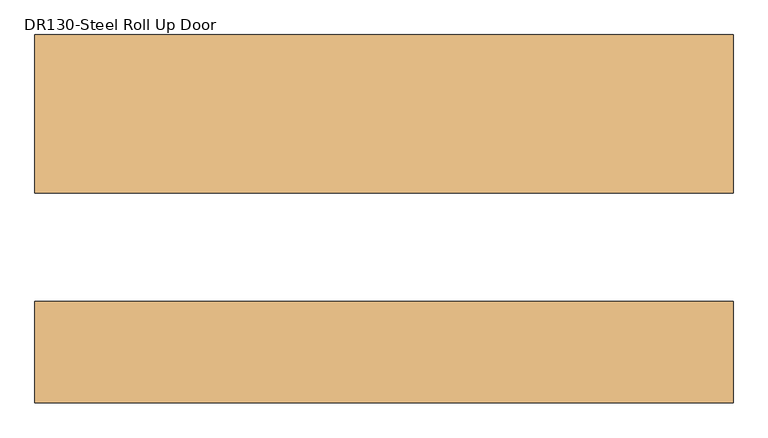
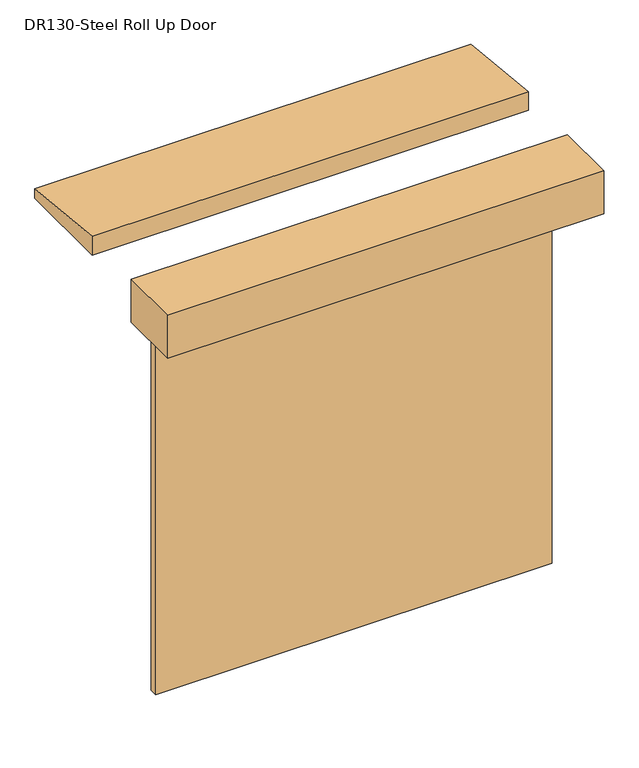
"""IFC4 building model written with IfcOpenShell, lengths in millimetres: door geometry, DR130-Steel Roll Up Door : DR131-Steel Roll Up Door-W4000xH4000mm."""

from ifc_helpers import new_model, si_unit, frame, origin, origin_with_axes, place, context, project, spatial, polyline, outline, extrude, source, transform, mapped, element, save


def dr130_steel_roll_up_door_abb043e2(model_context):
    return source(origin(), model_context, "Body", "SweptSolid", [
        extrude(outline(polyline([(1175.0, 4300.0), (175.0, 4300.0), (175.0, 4500.0), (1175.0, 4400.0), (1175.0, 4300.0)])), frame((-2203.2, 0.0, 0.0), z_axis=(1.0, 0.0, 0.0), x_axis=(0.0, 1.0, 0.0)), (0.0, 0.0, 1.0), 4406.4),
        extrude(outline(polyline([(2203.2, -1148.8), (-2203.2, -1148.8), (-2203.2, -510.0), (2203.2, -510.0), (2203.2, -1148.8)])), frame((0.0, 0.0, 4000.0), z_axis=(0.0, 0.0, 1.0), x_axis=(1.0, 0.0, 0.0)), (0.0, 0.0, 1.0), 457.2),
        extrude(outline(polyline([(2000.0, -510.0), (2000.0, -590.0), (-2000.0, -590.0), (-2000.0, -510.0), (2000.0, -510.0)])), origin_with_axes(), (0.0, 0.0, 1.0), 4000.0),
    ])


if __name__ == "__main__":
    model = new_model("IFC4")
    model_context = context("Model", 3, world=origin())
    ifc_project = project(units=[si_unit("LENGTHUNIT", "METRE", prefix="MILLI")], contexts=[model_context])
    site = spatial("IfcSite", under=ifc_project)
    building = spatial("IfcBuilding", under=site)
    placement = place(None, origin())
    dr130_steel_roll_up_door_shape = dr130_steel_roll_up_door_abb043e2(model_context)
    element("IfcDoor", 1, ObjectType="DR130-Steel Roll Up Door : DR131-Steel Roll Up Door-W4000xH4000mm", at=placement, inside=building, context=model_context, shape_type="MappedRepresentation", body=[
        mapped(dr130_steel_roll_up_door_shape, transform((0.0, 0.0, 0.0), x_axis=(1.0, 0.0, 0.0), y_axis=(0.0, 1.0, 0.0), z_axis=(0.0, 0.0, 1.0))),
    ])
    save(model, "model.ifc")

# Revit data of these elements
# Type "DR130-Steel Roll Up Door : DR131-Steel Roll Up Door-W4000xH4000mm"
#   Type Mark = "361"
#   Construction Type Id = "MDOOR"
#   Assembly Code = "B2030400"
#   Analytic Construction = "<None>"
#   Thickness = 80 mm
#   Thermal Resistance (R) = 0.270117 (m²·K)/W
#   Rough Width [instance default] = 4000 mm
#   Rough Height [instance default] = 4000 mm
#   Offset [instance default] = 1000 mm
#   Heat Transfer Coefficient (U) = 3.7021 W/(m²·K)
#   Height [instance default] = 4000 mm
#   Width [instance default] = 4000 mm
#   Function = 1
#   Define Thermal Properties by = 1
#   Canopy [instance default] = yes
#   Roller Material = A04AQ112-00002_Steel Roll Up Door
#   Roller Box Material = A04AQ112-00002_Steel Roll Up Door
#   Visual Light Transmittance = 0
#   Solar Heat Gain Coefficient = 0
#   Wall Closure = (empty or 0)
# Element 1 (IfcDoor, "DR130-Steel Roll Up Door : DR131-Steel Roll Up Door-W4000xH4000mm")
#   Offset = 550 mm
#   Materials on its faces: "A04AQ112-00002_Steel Roll Up Door"
# Materials
#   "A04AQ112-00002_Steel Roll Up Door": class "금속", colour RGB 247 247 247, transparency 0, Description = "Steel Door", W00) Work Master Code = "A04AQ112-00002", W01) Work Master_Lv1 = "Finishing Work", W02) Work Master_Lv2 = "Door & Window Work", W03) Work Master_Spec.1 = "Steel Roll Up Door w/ Steel Frame", W04) Work Master_Spec.2 = "Fire Protective Rating: N/A, Motorized Type", W05) Work Master_Spec.3 = "w/ Hardware & Accessories", Cost = 0
